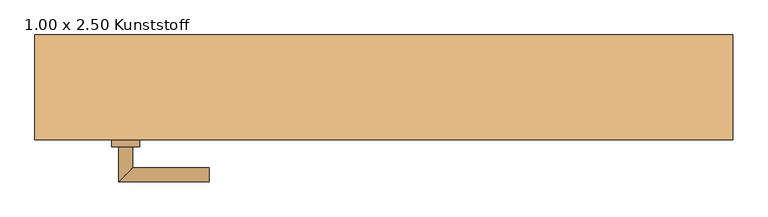
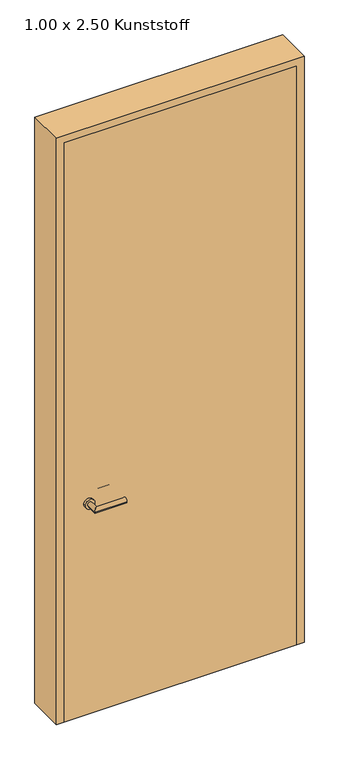
"""IFC4 building model written with IfcOpenShell, lengths in millimetres: door geometry, Drehflügel 1-flg - Blockzarge : 1.00 x 2.50 Kunststoff."""

from ifc_helpers import new_model, si_unit, point, frame, frame_2d, origin, place, context, project, spatial, polyline, circle_curve, ellipse_curve, trimmed, segment, composite_curve, outline, extrude, source, transform, mapped, element, save
from ifc_brep_helpers import plane_surface, cylinder_surface, advanced_brep


def door_1_00_x_2_50_kunststoff_a895dbe0(model_context):
    return source(origin(), model_context, "Body", "SolidModel", [
        advanced_brep(
        [(-360.0, -54.4346141, 1000.0), (-380.0, -54.4346141, 1000.0), (-380.0, -4.4346141, 1000.0), (-360.0, -24.4346141, 1000.0), (-250.0, -24.4346141, 1000.0), (-250.0, -4.4346141, 1000.0)],
        [
            (0, 1, circle_curve(frame((-370.0, -54.4346141, 1000.0), z_axis=(0.0, -1.0, 0.0), x_axis=(-1.0, 0.0, 0.0)), 10.0)),
            (1, 0, circle_curve(frame((-370.0, -54.4346141, 1000.0), z_axis=(0.0, -1.0, 0.0), x_axis=(-1.0, 0.0, 0.0)), 10.0)),
            (1, 2),
            (2, 3, ellipse_curve(frame((-370.0, -14.4346141, 1000.0), z_axis=(-0.7071067811865686, -0.7071067811865265, 0.0), x_axis=(0.7071067811865264, -0.7071067811865687, 0.0)), 14.1421356, 10.0)),
            (3, 0),
            (3, 2, ellipse_curve(frame((-370.0, -14.4346141, 1000.0), z_axis=(-0.7071067811865686, -0.7071067811865265, 0.0), x_axis=(0.7071067811865264, -0.7071067811865687, 0.0)), 14.1421356, 10.0)),
            (4, 5, circle_curve(frame((-250.0, -14.4346141, 1000.0), z_axis=(1.0, 0.0, 0.0), x_axis=(0.0, 1.0, 0.0)), 10.0)),
            (5, 4, circle_curve(frame((-250.0, -14.4346141, 1000.0), z_axis=(1.0, 0.0, 0.0), x_axis=(0.0, 1.0, 0.0)), 10.0)),
            (2, 5),
            (4, 3),
        ],
        [
            plane_surface(frame((-370.0, -54.4346141, -287.7526403), z_axis=(0.0, -1.0, 0.0), x_axis=(0.0, 0.0, 1.0))),
            cylinder_surface(frame((-370.0, -54.4346141, 1000.0), z_axis=(0.0, -1.0, 0.0), x_axis=(-1.0, 0.0, 0.0)), 10.0),
            plane_surface(frame((-250.0, -14.4346141, -287.7526403), z_axis=(1.0, 0.0, 0.0), x_axis=(0.0, 0.0, 1.0))),
            cylinder_surface(frame((-370.0, -14.4346141, 1000.0), z_axis=(-1.0, 0.0, 0.0), x_axis=(0.0, 1.0, 0.0)), 10.0),
        ],
        [
            (0, [[1, 2]]),
            (1, [[3, 4, 5, -2]]),
            (1, [[-5, 6, -3, -1]]),
            (2, [[7, 8]]),
            (3, [[9, -7, 10, -4]]),
            (3, [[-10, -8, -9, -6]]),
        ],
    ),
        advanced_brep(
        [(-360.0, -99.4346141, 1000.0), (-380.0, -99.4346141, 1000.0), (-380.0, -149.4346141, 1000.0), (-360.0, -129.4346141, 1000.0), (-250.0, -129.4346141, 1000.0), (-250.0, -149.4346141, 1000.0)],
        [
            (0, 1, circle_curve(frame((-370.0, -99.4346141, 1000.0), z_axis=(0.0, 1.0, 0.0), x_axis=(-1.0, 0.0, 0.0)), 10.0)),
            (1, 0, circle_curve(frame((-370.0, -99.4346141, 1000.0), z_axis=(0.0, 1.0, 0.0), x_axis=(-1.0, 0.0, 0.0)), 10.0)),
            (1, 2),
            (2, 3, ellipse_curve(frame((-370.0, -139.4346141, 1000.0), z_axis=(-0.7071067811865486, 0.7071067811865464, 0.0), x_axis=(0.7071067811865464, 0.7071067811865488, 0.0)), 14.1421356, 10.0)),
            (3, 0),
            (3, 2, ellipse_curve(frame((-370.0, -139.4346141, 1000.0), z_axis=(-0.7071067811865486, 0.7071067811865464, 0.0), x_axis=(0.7071067811865464, 0.7071067811865488, 0.0)), 14.1421356, 10.0)),
            (4, 5, circle_curve(frame((-250.0, -139.4346141, 1000.0), z_axis=(1.0, 0.0, 0.0), x_axis=(0.0, -1.0, 0.0)), 10.0)),
            (5, 4, circle_curve(frame((-250.0, -139.4346141, 1000.0), z_axis=(1.0, 0.0, 0.0), x_axis=(0.0, -1.0, 0.0)), 10.0)),
            (2, 5),
            (4, 3),
        ],
        [
            plane_surface(frame((-370.0, -99.4346141, -287.7526403), z_axis=(0.0, 1.0, 0.0), x_axis=(0.0, 0.0, 1.0))),
            cylinder_surface(frame((-370.0, -99.4346141, 1000.0), z_axis=(0.0, 1.0, 0.0), x_axis=(-1.0, 0.0, 0.0)), 10.0),
            plane_surface(frame((-250.0, -139.4346141, -287.7526403), z_axis=(1.0, 0.0, 0.0), x_axis=(0.0, 0.0, 1.0))),
            cylinder_surface(frame((-370.0, -139.4346141, 1000.0), z_axis=(-1.0, 0.0, 0.0), x_axis=(0.0, -1.0, 0.0)), 10.0),
        ],
        [
            (0, [[1, 2]]),
            (1, [[3, 4, 5, -2]]),
            (1, [[-5, 6, -3, -1]]),
            (2, [[7, 8]]),
            (3, [[9, -7, 10, -4]]),
            (3, [[-10, -8, -9, -6]]),
        ],
    ),
        extrude(outline(composite_curve([segment(trimmed(circle_curve(frame_2d((1000.0, -370.0)), 20.0), [point((1000.0, -350.0))], [point((1000.0, -390.0))], False, "CARTESIAN"), True, "CONTINUOUS"), segment(trimmed(circle_curve(frame_2d((1000.0, -370.0)), 20.0), [point((1000.0, -390.0))], [point((1000.0, -350.0))], False, "CARTESIAN"), True, "CONTINUOUS")], self_intersect=False)), frame((0.0, -64.4346141, 0.0), z_axis=(0.0, 1.0, 0.0), x_axis=(0.0, 0.0, 1.0)), (0.0, 0.0, 1.0), 10.0),
        extrude(outline(composite_curve([segment(trimmed(circle_curve(frame_2d((1000.0, -370.0)), 20.0), [point((1000.0, -350.0))], [point((1000.0, -390.0))], False, "CARTESIAN"), True, "CONTINUOUS"), segment(trimmed(circle_curve(frame_2d((1000.0, -370.0)), 20.0), [point((1000.0, -390.0))], [point((1000.0, -350.0))], False, "CARTESIAN"), True, "CONTINUOUS")], self_intersect=False)), frame((0.0, -99.4346141, 0.0), z_axis=(0.0, 1.0, 0.0), x_axis=(0.0, 0.0, 1.0)), (0.0, 0.0, 1.0), 10.0),
        extrude(outline(polyline([(2600.0, 500.0), (2600.0, -500.0), (100.0, -500.0), (100.0, -470.0), (2570.0, -470.0), (2570.0, 470.0), (100.0, 470.0), (100.0, 500.0), (2600.0, 500.0)])), frame((0.0, -89.4346141, 0.0), z_axis=(0.0, 1.0, 0.0), x_axis=(0.0, 0.0, 1.0)), (0.0, 0.0, 1.0), 150.0),
        extrude(outline(polyline([(470.0, -89.4346141), (-470.0, -89.4346141), (-470.0, -64.4346141), (470.0, -64.4346141), (470.0, -89.4346141)])), frame((0.0, 0.0, 100.0), z_axis=(0.0, 0.0, 1.0), x_axis=(1.0, 0.0, 0.0)), (0.0, 0.0, 1.0), 2470.0),
    ])


if __name__ == "__main__":
    model = new_model("IFC4")
    model_context = context("Model", 3, world=origin())
    ifc_project = project(units=[si_unit("LENGTHUNIT", "METRE", prefix="MILLI")], contexts=[model_context])
    site = spatial("IfcSite", under=ifc_project)
    building = spatial("IfcBuilding", under=site)
    placement = place(None, origin())
    door_1_00_x_2_50_kunststoff_shape = door_1_00_x_2_50_kunststoff_a895dbe0(model_context)
    element("IfcDoor", 1, ObjectType="Drehflügel 1-flg - Blockzarge : 1.00 x 2.50 Kunststoff", at=placement, inside=building, context=model_context, shape_type="MappedRepresentation", body=[
        mapped(door_1_00_x_2_50_kunststoff_shape, transform((0.0, 0.0, 0.0), x_axis=(1.0, 0.0, 0.0), y_axis=(0.0, 1.0, 0.0), z_axis=(0.0, 0.0, 1.0))),
    ])
    save(model, "model.ifc")

# Revit data of these elements
# Type "Drehflügel 1-flg - Blockzarge : 1.00 x 2.50 Kunststoff"
#   Type Mark = "25"
#   Operation = "SingleSwingRight"
#   Keynote = "16.03"
#   Visual Light Transmittance = 0.9
#   Solar Heat Gain Coefficient = 0.86
#   Heat Transfer Coefficient (U) = 5.5617 W/(m²·K)
#   Rough Width = 1.000 m
#   Stärke Futter = 0.030 m
#   Rough Height [instance default] = 2.600 m
#   Höhe Türgriff = 0.900 m
#   Height = 2.500 m
#   Fußbodenaufbau [instance default] = 0.100 m
#   Width = 1.000 m
#   Sichtbarkeit Sturzlinien [instance default] = yes
#   Türgriff auswählen [instance default] = element 420047
#   Türgriff [instance default] = none
#   Türflügel [instance default] = none
#   Rahmen/Pfosten [instance default] = none
#   Construction Type Id = ""
#   Function = (empty or 0)
#   Wall Closure = (empty or 0)
#   Analytic Construction = (empty or 0)
# Element 1 (IfcDoor, "Drehflügel 1-flg - Blockzarge : 1.00 x 2.50 Kunststoff")
#   Türflügel = Kunststoff
#   Rahmen/Pfosten = Kunststoff
#   Materials on its faces: "Metall - Chrom", "Kunststoff"
# Materials
#   "Metall - Chrom": class "Metall", colour RGB 247 247 247, transparency 0, Cost = 0
#   "Kunststoff": class "Allgemeines", colour RGB 0 0 0, transparency 0, Cost = 0
